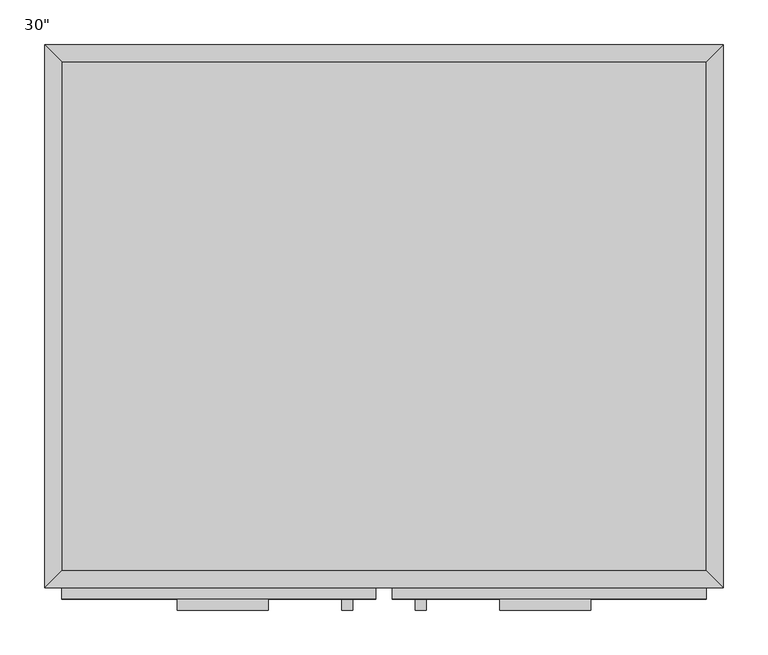
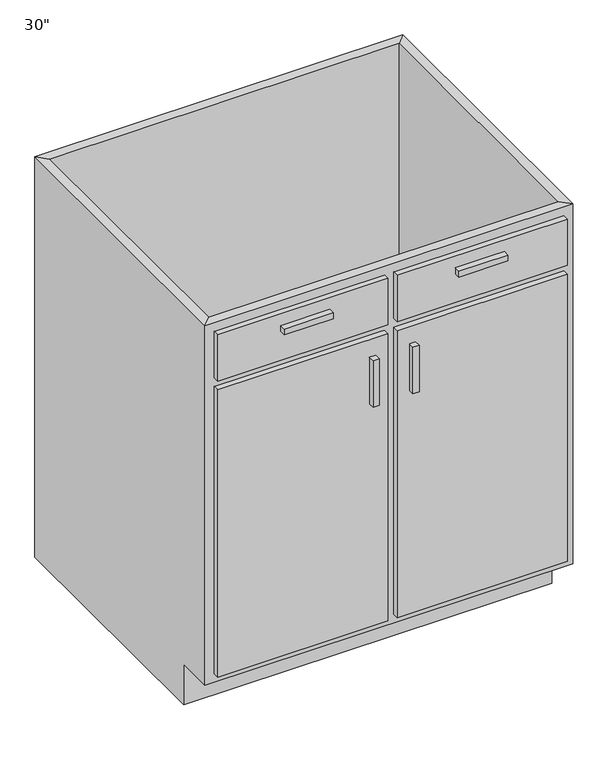
"""IFC4 building model written with IfcOpenShell, lengths in millimetres: furniture geometry."""

import ifcopenshell
import ifcopenshell.guid

model = None  # the IFC model being written
_history = None  # IfcOwnerHistory: only IFC2X3 demands one
_inside = {}  # id of a spatial element -> (the spatial element, [elements in it])
_under = {}  # id of a project, library or spatial element -> (it, [spatial elements below it])
_declared = {}  # id of a project -> (the project, [libraries it declares])
_typed = {}  # id of a type object -> (the type object, [elements of that type])
_made_of = {}  # id of a material, layer set ... -> (it, [elements and type objects made of it])


def new_model(schema):
    """Start an empty IFC model of exactly this schema.

    Asked for "IFC4X3", IfcOpenShell would pick the latest addendum, in which some entities
    have other attributes; the version numbers below select the first issue.
    IFC2X3 requires an IfcOwnerHistory on every rooted entity: one is made here for all.
    """
    global model, _history
    if schema == "IFC4X3":
        model = ifcopenshell.file(schema_version=(4, 3, 0, 0))
    else:
        model = ifcopenshell.file(schema=schema)
    _inside.clear()
    _under.clear()
    _declared.clear()
    _typed.clear()
    _made_of.clear()
    _history = None
    if model.schema == "IFC2X3":
        org = make("IfcOrganization", Name="unknown")
        user = make(
            "IfcPersonAndOrganization",
            ThePerson=make("IfcPerson", FamilyName="unknown"),
            TheOrganization=org,
        )
        app = make(
            "IfcApplication",
            ApplicationDeveloper=org,
            Version="unknown",
            ApplicationFullName="unknown",
            ApplicationIdentifier="unknown",
        )
        _history = make(
            "IfcOwnerHistory",
            OwningUser=user,
            OwningApplication=app,
            ChangeAction="ADDED",
            CreationDate=0,
        )
    return model


def make(cls, **values):
    """One entity of the class cls with the attributes given. An attribute that is None is left unset."""
    return model.create_entity(
        cls, **{name: value for name, value in values.items() if value is not None}
    )


def rooted(cls, **values):
    """An entity with a GlobalId (a new one), such as an element, a storey or a relation."""
    return make(cls, GlobalId=ifcopenshell.guid.new(), OwnerHistory=_history, **values)


def si_unit(unit_type, name, prefix=None):
    """IfcSIUnit, for example si_unit("LENGTHUNIT", "METRE", prefix="MILLI")."""
    return make("IfcSIUnit", UnitType=unit_type, Prefix=prefix, Name=name)


def assignment(units):
    """IfcUnitAssignment: the units of a project."""
    return None if units is None else make("IfcUnitAssignment", Units=units)


def point(xyz):
    """IfcCartesianPoint."""
    return None if xyz is None else make("IfcCartesianPoint", Coordinates=xyz)


def direction(xyz):
    """IfcDirection."""
    return None if xyz is None else make("IfcDirection", DirectionRatios=xyz)


def frame(location, z_axis=None, x_axis=None):
    """IfcAxis2Placement3D, a coordinate frame: its origin and axes. An axis left out is left unset."""
    return make(
        "IfcAxis2Placement3D",
        Location=point(location),
        Axis=direction(z_axis),
        RefDirection=direction(x_axis),
    )


def origin():
    """The frame at (0, 0, 0) with its axes left unset."""
    return frame((0.0, 0.0, 0.0))


def place(relative_to, where):
    """IfcLocalPlacement: puts the frame where relative to a parent placement (None: the world)."""
    return make(
        "IfcLocalPlacement", PlacementRelTo=relative_to, RelativePlacement=where
    )


def context(
    kind, dimensions, precision=None, world=None, true_north=None, identifier=None
):
    """IfcGeometricRepresentationContext, for example the 3D "Model" context."""
    return make(
        "IfcGeometricRepresentationContext",
        ContextIdentifier=identifier,
        ContextType=kind,
        CoordinateSpaceDimension=dimensions,
        Precision=precision,
        WorldCoordinateSystem=world,
        TrueNorth=true_north,
    )


def project(units=None, contexts=None):
    """IfcProject with its units and contexts."""
    return rooted(
        "IfcProject",
        Name="project",
        RepresentationContexts=contexts,
        UnitsInContext=assignment(units),
    )


def spatial(cls, under=None, at=None, **own):
    """A site, building, storey or space (cls), placed at a placement, below another one or the project."""
    s = rooted(cls, ObjectPlacement=at, **own)
    if under is not None:
        _under.setdefault(under.id(), (under, []))[1].append(s)
    return s


def polyline(points):
    """IfcPolyline through the points."""
    return make("IfcPolyline", Points=[point(p) for p in points])


def outline(outer, holes=None, kind="AREA"):
    """IfcArbitraryClosedProfileDef: a profile drawn as a closed curve; with holes, ...WithVoids."""
    if holes is None:
        return make("IfcArbitraryClosedProfileDef", ProfileType=kind, OuterCurve=outer)
    return make(
        "IfcArbitraryProfileDefWithVoids",
        ProfileType=kind,
        OuterCurve=outer,
        InnerCurves=holes,
    )


def extrude(swept, where, along, depth):
    """IfcExtrudedAreaSolid: the profile swept, set in the frame where, extruded along a direction by depth."""
    return make(
        "IfcExtrudedAreaSolid",
        SweptArea=swept,
        Position=where,
        ExtrudedDirection=direction(along),
        Depth=depth,
    )


def faces_of(points, faces, orient=None, outer=None):
    """IfcFace entities. A face is a list of loops; a loop is a list of indices into points, from 0.

    orient and outer hold one flag for each loop. By default every Orientation is true, the
    first loop of a face is its IfcFaceOuterBound and the others are IfcFaceBound.
    """
    made = []
    for i, loops in enumerate(faces):
        bounds = []
        for j, loop in enumerate(loops):
            is_outer = j == 0 if outer is None else outer[i][j]
            bounds.append(
                make(
                    "IfcFaceOuterBound" if is_outer else "IfcFaceBound",
                    Bound=make("IfcPolyLoop", Polygon=[points[k] for k in loop]),
                    Orientation=True if orient is None else orient[i][j],
                )
            )
        made.append(make("IfcFace", Bounds=bounds))
    return made


def faceted_brep(points, faces, orient=None, outer=None, voids=None):
    """IfcFacetedBrep: a solid bounded by flat faces; with voids (closed shells), ...WithVoids."""
    shared = [point(p) for p in points]
    hull = make("IfcClosedShell", CfsFaces=faces_of(shared, faces, orient, outer))
    if voids is None:
        return make("IfcFacetedBrep", Outer=hull)
    return make(
        "IfcFacetedBrepWithVoids",
        Outer=hull,
        Voids=[
            make(cls, CfsFaces=faces_of(shared, fs, o, b)) for cls, fs, o, b in voids
        ],
    )


def shape(context_of_items, identifier, shape_type, items):
    """IfcShapeRepresentation: the items that make up one representation, for example the "Body"."""
    return make(
        "IfcShapeRepresentation",
        ContextOfItems=context_of_items,
        RepresentationIdentifier=identifier,
        RepresentationType=shape_type,
        Items=items,
    )


def source(mapping_origin, context_of_items, identifier, shape_type, items):
    """IfcRepresentationMap: a shape defined once, which mapped items show again and again."""
    return make(
        "IfcRepresentationMap",
        MappingOrigin=mapping_origin,
        MappedRepresentation=shape(context_of_items, identifier, shape_type, items),
    )


def transform(
    local_origin,
    x_axis=None,
    y_axis=None,
    z_axis=None,
    scale=None,
    scale2=None,
    scale3=None,
    uniform=True,
):
    """IfcCartesianTransformationOperator3D, or its non-uniform kind. x_axis, y_axis, z_axis: its Axis1, 2, 3."""
    if uniform:
        return make(
            "IfcCartesianTransformationOperator3D",
            Axis1=direction(x_axis),
            Axis2=direction(y_axis),
            LocalOrigin=point(local_origin),
            Scale=scale,
            Axis3=direction(z_axis),
        )
    return make(
        "IfcCartesianTransformationOperator3DnonUniform",
        Axis1=direction(x_axis),
        Axis2=direction(y_axis),
        LocalOrigin=point(local_origin),
        Scale=scale,
        Axis3=direction(z_axis),
        Scale2=scale2,
        Scale3=scale3,
    )


def mapped(mapping_source, mapping_target):
    """IfcMappedItem: shows the shape of a source again, moved by a transform."""
    return make(
        "IfcMappedItem", MappingSource=mapping_source, MappingTarget=mapping_target
    )


def made_of(thing, what):
    """Note that an element or type object is made of a material, layer set ...; save() writes the relation."""
    if what is not None:
        _made_of.setdefault(what.id(), (what, []))[1].append(thing)
    return thing


def element(
    cls,
    number,
    at=None,
    inside=None,
    cuts=None,
    type_object=None,
    material=None,
    context=None,
    identifier="Body",
    shape_type=None,
    held_by="IfcProductDefinitionShape",
    body=None,
    shapes=None,
    **own,
):
    """One element of the class cls, such as IfcWall. Its Tag is "e" and its number.

    at: its placement. inside: the storey or other place that contains it. cuts: it is an
    opening in that element (IfcRelVoidsElement). A single representation is given by context,
    identifier, shape_type and body (its items); several are given by shapes. held_by: the class
    of the entity that holds the representations. save() writes the other relations.
    """
    e = rooted(cls, Tag="e%d" % number, ObjectPlacement=at, **own)
    if body is not None:
        shapes = [shape(context, identifier, shape_type, body)]
    if shapes is not None:
        e.Representation = make(held_by, Representations=shapes)
    if inside is not None:
        _inside.setdefault(inside.id(), (inside, []))[1].append(e)
    if cuts is not None:
        rooted(
            "IfcRelVoidsElement", RelatingBuildingElement=cuts, RelatedOpeningElement=e
        )
    if type_object is not None:
        _typed.setdefault(type_object.id(), (type_object, []))[1].append(e)
    return made_of(e, material)


def aggregate(whole, parts):
    """IfcRelAggregates: a whole, such as a stair, and the parts it consists of."""
    return rooted("IfcRelAggregates", RelatingObject=whole, RelatedObjects=parts)


def save(model, path):
    """Write the relations noted so far, then the file.

    IfcRelAggregates (storeys below a building ...), IfcRelContainedInSpatialStructure (elements
    in a storey), IfcRelDefinesByType, IfcRelAssociatesMaterial and IfcRelDeclares: one each for
    every whole, place, type object, material and project.
    """
    for whole, parts in _under.values():
        aggregate(whole, parts)
    for where, things in _inside.values():
        rooted(
            "IfcRelContainedInSpatialStructure",
            RelatedElements=things,
            RelatingStructure=where,
        )
    for kind, things in _typed.values():
        rooted("IfcRelDefinesByType", RelatedObjects=things, RelatingType=kind)
    for what, things in _made_of.values():
        rooted("IfcRelAssociatesMaterial", RelatedObjects=things, RelatingMaterial=what)
    for by, libraries in _declared.values():
        rooted("IfcRelDeclares", RelatingContext=by, RelatedDefinitions=libraries)
    model.write(path)


def furniture_338da5bd(model_context):
    return source(origin(), model_context, "Body", "SolidModel", [
        faceted_brep([(380.6877049, -590.55, 876.3), (380.6877049, -590.55, 88.9), (-343.2122951, -590.55, 88.9), (-343.2122951, -590.55, 876.3), (-362.2622951, -609.6, 876.3), (399.7377049, -609.6, 876.3), (-362.2622951, -609.6, 88.9), (399.7377049, -609.6, 88.9), (-343.2122951, -533.4, 88.9), (-343.2122951, -19.05, 88.9), (-343.2122951, -19.05, 876.3), (-362.2622951, 0.0, 876.3), (-362.2622951, 0.0, 0.0), (-362.2622951, -533.4, 0.0), (-362.2622951, -533.4, 88.9), (380.6877049, -19.05, 88.9), (380.6877049, -19.05, 876.3), (399.7377049, 0.0, 876.3), (399.7377049, 0.0, 0.0), (380.6877049, -533.4, 88.9), (399.7377049, -533.4, 88.9), (399.7377049, -533.4, 0.0)], [[[0, 1, 2, 3]], [[0, 3, 4, 5]], [[5, 4, 6, 7]], [[2, 1, 7, 6]], [[3, 2, 8, 9, 10]], [[4, 3, 10, 11]], [[6, 4, 11, 12, 13, 14]], [[2, 6, 14, 8]], [[10, 9, 15, 16]], [[11, 10, 16, 17]], [[12, 11, 17, 18]], [[1, 0, 16, 15, 19]], [[0, 5, 17, 16]], [[5, 7, 20, 21, 18, 17]], [[7, 1, 19, 20]], [[8, 19, 15, 9]], [[18, 21, 13, 12]], [[13, 21, 20, 19, 8, 14]]]),
        extrude(outline(polyline([(-111.4372951, -635.0), (-213.0372951, -635.0), (-213.0372951, -622.3), (-111.4372951, -622.3), (-111.4372951, -635.0)])), frame((0.0, 0.0, 819.15), z_axis=(0.0, 0.0, 1.0), x_axis=(1.0, 0.0, 0.0)), (0.0, 0.0, 1.0), 12.7),
        extrude(outline(polyline([(250.5127049, -635.0), (148.9127049, -635.0), (148.9127049, -622.3), (250.5127049, -622.3), (250.5127049, -635.0)])), frame((0.0, 0.0, 819.15), z_axis=(0.0, 0.0, 1.0), x_axis=(1.0, 0.0, 0.0)), (0.0, 0.0, 1.0), 12.7),
        extrude(outline(polyline([(-16.1872951, -635.0), (-28.8872951, -635.0), (-28.8872951, -622.3), (-16.1872951, -622.3), (-16.1872951, -635.0)])), frame((0.0, 0.0, 596.9), z_axis=(0.0, 0.0, 1.0), x_axis=(1.0, 0.0, 0.0)), (0.0, 0.0, 1.0), 101.6),
        extrude(outline(polyline([(66.3627049, -635.0), (53.6627049, -635.0), (53.6627049, -622.3), (66.3627049, -622.3), (66.3627049, -635.0)])), frame((0.0, 0.0, 596.9), z_axis=(0.0, 0.0, 1.0), x_axis=(1.0, 0.0, 0.0)), (0.0, 0.0, 1.0), 101.6),
        extrude(outline(polyline([(380.6877049, -19.05), (380.6877049, -590.55), (-343.2122951, -590.55), (-343.2122951, -19.05), (380.6877049, -19.05)])), frame((0.0, 0.0, 88.9), z_axis=(0.0, 0.0, 1.0), x_axis=(1.0, 0.0, 0.0)), (0.0, 0.0, 1.0), 19.05),
        extrude(outline(polyline([(9.2127049, -622.3), (-343.2122951, -622.3), (-343.2122951, -609.6), (9.2127049, -609.6), (9.2127049, -622.3)])), frame((0.0, 0.0, 755.65), z_axis=(0.0, 0.0, 1.0), x_axis=(1.0, 0.0, 0.0)), (0.0, 0.0, 1.0), 101.6),
        extrude(outline(polyline([(380.6877049, -622.3), (28.2627049, -622.3), (28.2627049, -609.6), (380.6877049, -609.6), (380.6877049, -622.3)])), frame((0.0, 0.0, 755.65), z_axis=(0.0, 0.0, 1.0), x_axis=(1.0, 0.0, 0.0)), (0.0, 0.0, 1.0), 101.6),
        extrude(outline(polyline([(9.2127049, -622.3), (-343.2122951, -622.3), (-343.2122951, -609.6), (9.2127049, -609.6), (9.2127049, -622.3)])), frame((0.0, 0.0, 107.95), z_axis=(0.0, 0.0, 1.0), x_axis=(1.0, 0.0, 0.0)), (0.0, 0.0, 1.0), 628.65),
        extrude(outline(polyline([(380.6877049, -622.3), (28.2627049, -622.3), (28.2627049, -609.6), (380.6877049, -609.6), (380.6877049, -622.3)])), frame((0.0, 0.0, 107.95), z_axis=(0.0, 0.0, 1.0), x_axis=(1.0, 0.0, 0.0)), (0.0, 0.0, 1.0), 628.65),
    ])


if __name__ == "__main__":
    model = new_model("IFC4")
    model_context = context("Model", 3, world=origin())
    ifc_project = project(units=[si_unit("LENGTHUNIT", "METRE", prefix="MILLI")], contexts=[model_context])
    site = spatial("IfcSite", under=ifc_project)
    building = spatial("IfcBuilding", under=site)
    placement = place(None, origin())
    furniture_shape = furniture_338da5bd(model_context)
    element("IfcFurniture", 1, ObjectType="Base Cabinet-Double Door & 2 Drawer : 30\"", at=placement, inside=building, context=model_context, shape_type="MappedRepresentation", body=[
        mapped(furniture_shape, transform((0.0, 0.0, 0.0), x_axis=(1.0, 0.0, 0.0), y_axis=(0.0, 1.0, 0.0), z_axis=(0.0, 0.0, 1.0))),
    ])
    save(model, "model.ifc")

# Revit data of these elements
# Type "Base Cabinet-Double Door & 2 Drawer : 30\""
#   Assembly Code = "C1030410"
#   Depth = 2' - 0"
#   Height = 2' - 10 1/2"
#   Toe Depth = 0' - 3"
#   Toe Height = 0' - 3 1/2"
#   Width = 2' - 6"
#   Cabinet Material = none
#   Door/Drawer Material = none
#   Handle Material = Cabinets - Handles
#   Default Elevation = 0
# Element 1 (IfcFurniture, "Base Cabinet-Double Door & 2 Drawer : 30\"")
#   Materials on its faces: "Cabinets", "Cabinets - Handles"
# Materials
#   "Cabinets - Handles": class "Metal", colour RGB 57 57 57, transparency 0
#   "Cabinets": class "Miscellaneous", colour RGB 249 249 249, transparency 0
